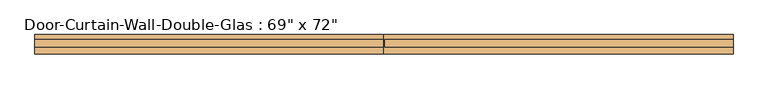
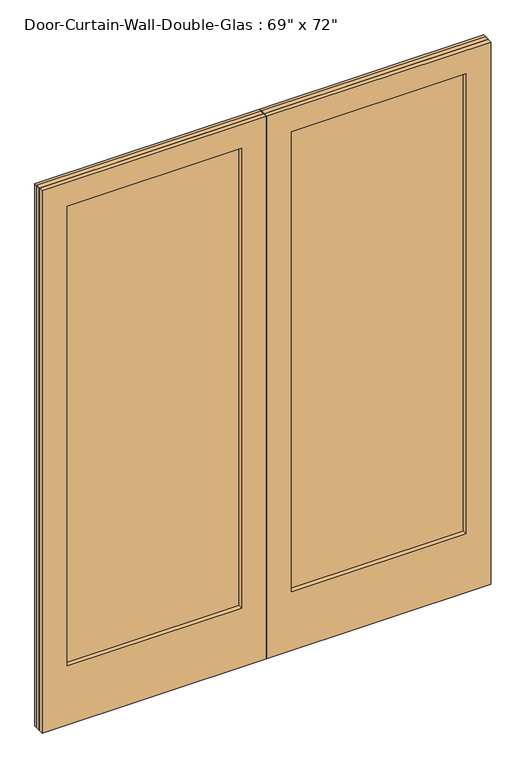
"""IFC4 building model written with IfcOpenShell, lengths in millimetres: door geometry."""

from ifc_helpers import new_model, si_unit, frame, origin, origin_with_axes, place, context, project, spatial, polyline, outline, extrude, source, transform, mapped, element, save


def door_8e8f9c27(model_context):
    return source(origin(), model_context, "Body", "SweptSolid", [
        extrude(outline(polyline([(915.9352729, 31.75), (1.5606001, 31.75), (1.5606001, 50.8), (915.9352729, 50.8), (915.9352729, 31.75)])), origin_with_axes(), (0.0, 0.0, 1.0), 2338.0),
        extrude(outline(polyline([(-1.6143999, 31.75), (-915.9352729, 31.75), (-915.9352729, 50.8), (-1.6143999, 50.8), (-1.6143999, 31.75)])), origin_with_axes(), (0.0, 0.0, 1.0), 2338.0),
        extrude(outline(polyline([(2338.0, -0.0268999), (0.0, -0.0268999), (0.0, 915.9352729), (2338.0, 915.9352729), (2338.0, -0.0268999)]), holes=[polyline([(2236.4, 101.5731001), (2236.4, 814.3352729), (254.0, 814.3352729), (254.0, 101.5731001), (2236.4, 101.5731001)])]), frame((0.0, 12.7, 0.0), z_axis=(0.0, 1.0, 0.0), x_axis=(0.0, 0.0, 1.0)), (0.0, 0.0, 1.0), 50.8),
        extrude(outline(polyline([(2338.0, -0.0268999), (2338.0, -915.9352729), (0.0, -915.9352729), (0.0, -0.0268999), (2338.0, -0.0268999)]), holes=[polyline([(2236.4, -101.6268999), (254.0, -101.6268999), (254.0, -814.3352729), (2236.4, -814.3352729), (2236.4, -101.6268999)])]), frame((0.0, 12.7, 0.0), z_axis=(0.0, 1.0, 0.0), x_axis=(0.0, 0.0, 1.0)), (0.0, 0.0, 1.0), 50.8),
    ])


if __name__ == "__main__":
    model = new_model("IFC4")
    model_context = context("Model", 3, world=origin())
    ifc_project = project(units=[si_unit("LENGTHUNIT", "METRE", prefix="MILLI")], contexts=[model_context])
    site = spatial("IfcSite", under=ifc_project)
    building = spatial("IfcBuilding", under=site)
    placement = place(None, origin())
    door_shape = door_8e8f9c27(model_context)
    element("IfcDoor", 1, ObjectType="Door-Curtain-Wall-Double-Glas : 69\" x 72\"", at=placement, inside=building, context=model_context, shape_type="MappedRepresentation", body=[
        mapped(door_shape, transform((0.0, 0.0, 0.0), x_axis=(1.0, 0.0, 0.0), y_axis=(0.0, 1.0, 0.0), z_axis=(0.0, 0.0, 1.0))),
    ])
    save(model, "model.ifc")

# Revit data of these elements
# Type "Door-Curtain-Wall-Double-Glas : 69\" x 72\""
#   Type Mark = "64"
#   ZGF Door Panel Type = "G2"
#   Panel Type = "G2"
#   Assembly Code = "B2030100"
#   Analytic Construction = "<None>"
#   Width [instance default] = 1828.8 mm
#   Thickness = 44.45 mm
#   Thermal Resistance (R) = 1.7611 (m²·K)/W
#   Swing Angle [instance default] = 90.00°
#   Panel Width [instance default] = 914.4 mm
#   Offset = 50.8 mm
#   Heat Transfer Coefficient (U) = 0.567826 W/(m²·K)
#   Code Exit Load Factor [instance default] = 0.2
#   Code Clear Width Reduction = 76.2 mm
#   Clear Width [instance default] = 1752.6 mm
#   CALC Imperial Conversion from Feet = 12
#   Door Frame = yes
#   Define Thermal Properties by = 1
#   Function = 1
#   Code Exit Load [instance default] = 0
#   Code Exit Capacity [instance default] = 345
#   Door Handle Material = PAE Metal Panel Dark****
#   Glazing = Glass
#   Visual Light Transmittance = 0
#   Solar Heat Gain Coefficient = 0
#   Construction Type Id = ""
# Element 1 (IfcDoor, "Door-Curtain-Wall-Double-Glas : 69\" x 72\"")
#   Width = 1831.871 mm
#   Panel Width = 915.935 mm
#   Clear Width = 1755.671 mm
#   Code Exit Capacity = 346
#   Materials on its faces: "PAE Cascadia Mullion", "Glass"
# Materials
#   "PAE Metal Panel Dark****": class "Generic", colour RGB 192 192 192, transparency 0, Keynote = "MP1", Description = "MP1", Cost = 0
#   "Glass": class "Glass", colour RGB 0 128 192, transparency 0.9, Description = "Soda Lime Glass", Cost = 0
#   "PAE Cascadia Mullion": class "Metal", colour RGB 120 120 120, transparency 0, Description = "Steel, paint finish, blue", Cost = 0
